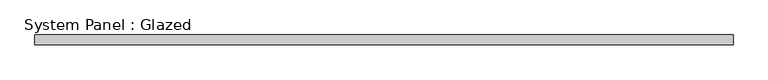
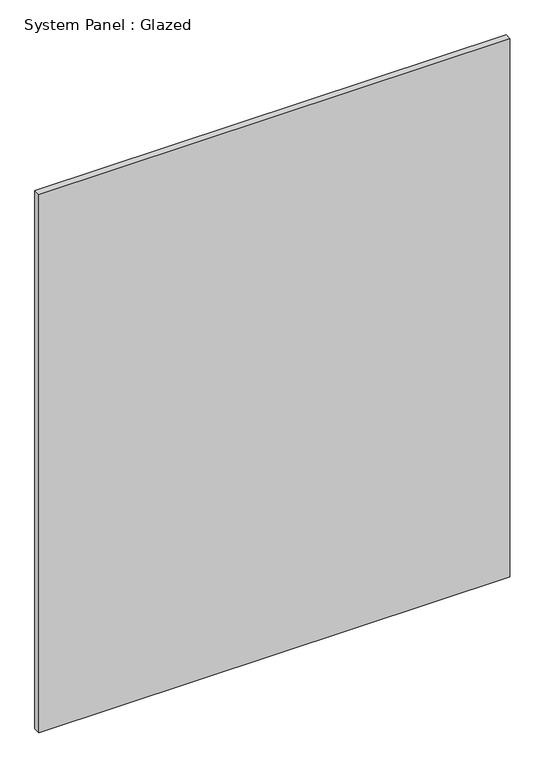
"""IFC4 building model written with IfcOpenShell, lengths in millimetres: plate geometry, System Panel : Glazed."""

from ifc_helpers import new_model, si_unit, origin, origin_with_axes, place, context, project, spatial, polyline, outline, extrude, source, transform, mapped, element, save


def system_panel_glazed_aeb7b79b(model_context):
    return source(origin(), model_context, "Body", "SweptSolid", [
        extrude(outline(polyline([(879.5, -49.5), (-879.5, -49.5), (-879.5, -24.5), (879.5, -24.5), (879.5, -49.5)])), origin_with_axes(), (0.0, 0.0, 1.0), 2125.0),
    ])


if __name__ == "__main__":
    model = new_model("IFC4")
    model_context = context("Model", 3, world=origin())
    ifc_project = project(units=[si_unit("LENGTHUNIT", "METRE", prefix="MILLI")], contexts=[model_context])
    site = spatial("IfcSite", under=ifc_project)
    building = spatial("IfcBuilding", under=site)
    placement = place(None, origin())
    system_panel_glazed_shape = system_panel_glazed_aeb7b79b(model_context)
    element("IfcPlate", 1, ObjectType="System Panel : Glazed", at=placement, inside=building, context=model_context, shape_type="MappedRepresentation", body=[
        mapped(system_panel_glazed_shape, transform((0.0, 0.0, 0.0), x_axis=(1.0, 0.0, 0.0), y_axis=(0.0, 1.0, 0.0), z_axis=(0.0, 0.0, 1.0))),
    ])
    save(model, "model.ifc")

# Revit data of these elements
# Type "System Panel : Glazed"
#   Keynote = "H11"
#   Construction Type Id = "GSP4R"
#   Analytic Construction = "1/8 in Pilkington single glazing"
#   Visual Light Transmittance = 0.9
#   Solar Heat Gain Coefficient = 0.86
#   Heat Transfer Coefficient (U) = 6.7069 W/(m²·K)
# Element 1 (IfcPlate, "System Panel : Glazed")
#   Materials on its faces: "Glass"
# Materials
#   "Glass": class "Glass", colour RGB 0 128 192, transparency 0.9, Description = "Soda Lime Glass", Cost = 0
